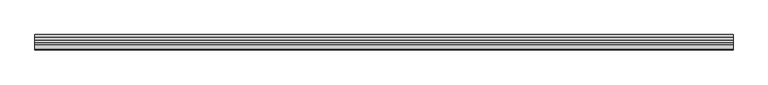
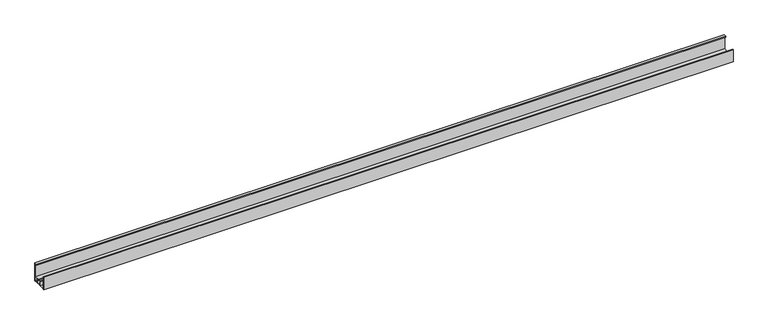
"""IFC4 building model written with IfcOpenShell, lengths in millimetres: proxy geometry, Generic Models 3:Generic Models 2:312240:Generic Models 2:312240 : Generic Models 3:Generic Models 2:312240:3 : Generic Models 3:Generic Models 2:312240:Generic Models 2:312240 : Generic Models 3:Generic Models 2:312240:300533."""

from ifc_helpers import new_model, si_unit, frame, origin, place, context, project, spatial, polyline, outline, extrude, source, transform, mapped, element, save


def generic_models_5224f214(model_context):
    return source(origin(), model_context, "Body", "SweptSolid", [
        extrude(outline(polyline([(-568250.385512, 4875.4957253), (-568233.8332558, 4875.4957253), (-568233.8332558, 4870.7982267), (-568235.7586712, 4870.7982267), (-568235.7586712, 4868.4169767), (-568233.8332558, 4868.4169767), (-568233.8332558, 4863.719478), (-568250.385512, 4863.719478), (-568250.385512, 4868.4169767), (-568248.4600965, 4868.4169767), (-568248.4600965, 4870.7982267), (-568250.385512, 4870.7982267), (-568250.385512, 4875.4957253)])), frame((591391.6367242, 0.0, 0.0), z_axis=(1.0, 0.0, 0.0), x_axis=(0.0, 1.0, 0.0)), (0.0, 0.0, 1.0), 2438.4),
        extrude(outline(polyline([(-568226.7958673, 4928.147603), (-568218.3494958, 4928.147603), (-568218.3494958, 4860.147603), (-568219.9369958, 4860.147603), (-568219.9369958, 4861.735103), (-568237.6035683, 4861.735103), (-568237.6035683, 4863.322603), (-568233.4363808, 4863.322603), (-568233.4363808, 4868.8138517), (-568235.3617962, 4868.8138517), (-568235.3617962, 4870.4013517), (-568233.4363808, 4870.4013517), (-568233.4363808, 4875.8926003), (-568237.6035683, 4875.8926003), (-568237.6035683, 4877.4801003), (-568219.9369958, 4877.4801003), (-568219.9369958, 4926.560103), (-568225.2083673, 4926.560103), (-568225.2083673, 4923.7602765), (-568226.7958673, 4923.7602765), (-568226.7958673, 4928.147603)]), holes=[polyline([(-568219.9369958, 4875.8926003), (-568231.8488808, 4875.8926003), (-568231.8488808, 4863.322603), (-568219.9369958, 4863.322603), (-568219.9369958, 4875.8926003)])]), frame((591391.6367242, 0.0, 0.0), z_axis=(1.0, 0.0, 0.0), x_axis=(0.0, 1.0, 0.0)), (0.0, 0.0, 1.0), 2438.4),
        extrude(outline(polyline([(-568270.7619958, 4860.147603), (-568272.3494958, 4860.147603), (-568272.3494958, 4906.1522905), (-568269.6344059, 4906.1522905), (-568269.6344059, 4904.5647905), (-568270.7619958, 4904.5647905), (-568270.7619958, 4863.322603), (-568252.369887, 4863.322603), (-568252.369887, 4877.4801003), (-568246.6151995, 4877.4801003), (-568246.6151995, 4875.8926003), (-568250.782387, 4875.8926003), (-568250.782387, 4870.4013517), (-568248.8569715, 4870.4013517), (-568248.8569715, 4868.8138517), (-568250.782387, 4868.8138517), (-568250.782387, 4863.322603), (-568246.6151995, 4863.322603), (-568246.6151995, 4861.735103), (-568270.7619958, 4861.735103), (-568270.7619958, 4860.147603)])), frame((591391.6367242, 0.0, 0.0), z_axis=(1.0, 0.0, 0.0), x_axis=(0.0, 1.0, 0.0)), (0.0, 0.0, 1.0), 2438.4),
    ])


if __name__ == "__main__":
    model = new_model("IFC4")
    model_context = context("Model", 3, world=origin())
    ifc_project = project(units=[si_unit("LENGTHUNIT", "METRE", prefix="MILLI")], contexts=[model_context])
    site = spatial("IfcSite", under=ifc_project)
    building = spatial("IfcBuilding", under=site)
    placement = place(None, origin())
    generic_models_shape = generic_models_5224f214(model_context)
    element("IfcBuildingElementProxy", 1, Name="Generic Models 3:Generic Models 2:312240:Generic Models 2:312240 : Generic Models 3:Generic Models 2:312240:3 : Generic Models 3:Generic Models 2:312240:Generic Models 2:312240 : Generic Models 3:Generic Models 2:312240:300533", ObjectType="Generic Models 3:Generic Models 2:312240:Generic Models 2:312240 : Generic Models 3:Generic Models 2:312240:3 : Generic Models 3:Generic Models 2:312240:Generic Models 2:312240 : Generic Models 3:Generic Models 2:312240:300533", at=placement, inside=building, context=model_context, shape_type="MappedRepresentation", body=[
        mapped(generic_models_shape, transform((0.0, 0.0, 0.0), x_axis=(1.0, 0.0, 0.0), y_axis=(0.0, 1.0, 0.0), z_axis=(0.0, 0.0, 1.0))),
    ])
    save(model, "model.ifc")

# Revit data of these elements
# Type "Generic Models 3:Generic Models 2:312240:Generic Models 2:312240 : Generic Models 3:Generic Models 2:312240:3 : Generic Models 3:Generic Models 2:312240:Generic Models 2:312240 : Generic Models 3:Generic Models 2:312240:300533"
#   NameOverride = "Generic Models 3:Generic Models 2:312240:Generic Models 2:312240 : Generic Models 3:Generic Models 2:312240:300533"
#   ObjectTypeOverride = "Generic Models 2:312240 : Generic Models 3:Generic Models 2:312240"
#   Reference = "Generic Models 2"
#   Tag = "300533"
# Element 1 (IfcBuildingElementProxy, "Generic Models 3:Generic Models 2:312240:Generic Models 2:312240 : Generic Models 3:Generic Models 2:312240:3 : Generic Models 3:Generic Models 2:312240:Generic Models 2:312240 : Generic Models 3:Generic Models 2:312240:300533")
#   Materials on its faces: "THERMAL BROKEN ALUMINUM STOREFRONT FOR POLYCARBONATE"
# Materials
#   "THERMAL BROKEN ALUMINUM STOREFRONT FOR POLYCARBONATE": class "Unassigned", colour RGB 244 244 244, transparency 0, Keynote = "M07611300.01", Cost = 0
